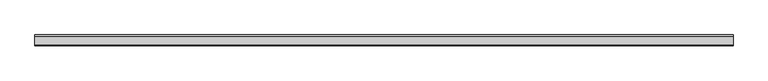
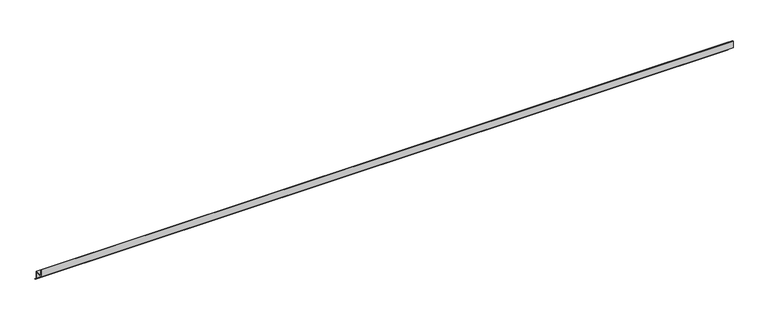
"""IFC4 building model written with IfcOpenShell, lengths in millimetres: proxy geometry, Generic Models 7:Generic Models 1:337419:Generic Models 1:337419 : Generic Models 7:Generic Models 1:337419:17 : Generic Models 7:Generic Models 1:337419:Generic Models 1:337419 : Generic Models 7:Generic Models 1:337419:301336."""

from ifc_helpers import new_model, si_unit, frame, origin, place, context, project, spatial, polyline, outline, extrude, source, transform, mapped, element, save


def generic_models_8e24153e(model_context):
    return source(origin(), model_context, "Body", "SweptSolid", [
        extrude(outline(polyline([(-566389.0516324, 4832.0490819), (-566389.0516324, 4882.8490819), (-566386.2735074, 4882.8490819), (-566386.2735074, 4834.8272069), (-566326.3453823, 4834.8272069), (-566326.3453823, 4784.0272069), (-566312.8749982, 4770.5568227), (-566314.8394292, 4768.5923917), (-566329.1235073, 4782.8764699), (-566329.1235073, 4832.0490819), (-566389.0516324, 4832.0490819)])), frame((597433.7867239, 0.0, 0.0), z_axis=(1.0, 0.0, 0.0), x_axis=(0.0, 1.0, 0.0)), (0.0, 0.0, 1.0), 4876.8),
    ])


if __name__ == "__main__":
    model = new_model("IFC4")
    model_context = context("Model", 3, world=origin())
    ifc_project = project(units=[si_unit("LENGTHUNIT", "METRE", prefix="MILLI")], contexts=[model_context])
    site = spatial("IfcSite", under=ifc_project)
    building = spatial("IfcBuilding", under=site)
    placement = place(None, origin())
    generic_models_shape = generic_models_8e24153e(model_context)
    element("IfcBuildingElementProxy", 1, Name="Generic Models 7:Generic Models 1:337419:Generic Models 1:337419 : Generic Models 7:Generic Models 1:337419:17 : Generic Models 7:Generic Models 1:337419:Generic Models 1:337419 : Generic Models 7:Generic Models 1:337419:301336", ObjectType="Generic Models 7:Generic Models 1:337419:Generic Models 1:337419 : Generic Models 7:Generic Models 1:337419:17 : Generic Models 7:Generic Models 1:337419:Generic Models 1:337419 : Generic Models 7:Generic Models 1:337419:301336", at=placement, inside=building, context=model_context, shape_type="MappedRepresentation", body=[
        mapped(generic_models_shape, transform((0.0, 0.0, 0.0), x_axis=(1.0, 0.0, 0.0), y_axis=(0.0, 1.0, 0.0), z_axis=(0.0, 0.0, 1.0))),
    ])
    save(model, "model.ifc")

# Revit data of these elements
# Type "Generic Models 7:Generic Models 1:337419:Generic Models 1:337419 : Generic Models 7:Generic Models 1:337419:17 : Generic Models 7:Generic Models 1:337419:Generic Models 1:337419 : Generic Models 7:Generic Models 1:337419:301336"
#   NameOverride = "Generic Models 7:Generic Models 1:337419:Generic Models 1:337419 : Generic Models 7:Generic Models 1:337419:301336"
#   ObjectTypeOverride = "Generic Models 1:337419 : Generic Models 7:Generic Models 1:337419"
#   Reference = "Generic Models 1"
#   Tag = "301336"
# Element 1 (IfcBuildingElementProxy, "Generic Models 7:Generic Models 1:337419:Generic Models 1:337419 : Generic Models 7:Generic Models 1:337419:17 : Generic Models 7:Generic Models 1:337419:Generic Models 1:337419 : Generic Models 7:Generic Models 1:337419:301336")
#   Materials on its faces: "BRAKE METAL FLASHING"
# Materials
#   "BRAKE METAL FLASHING": class "Unassigned", colour RGB 210 209 208, transparency 0, Cost = 0
